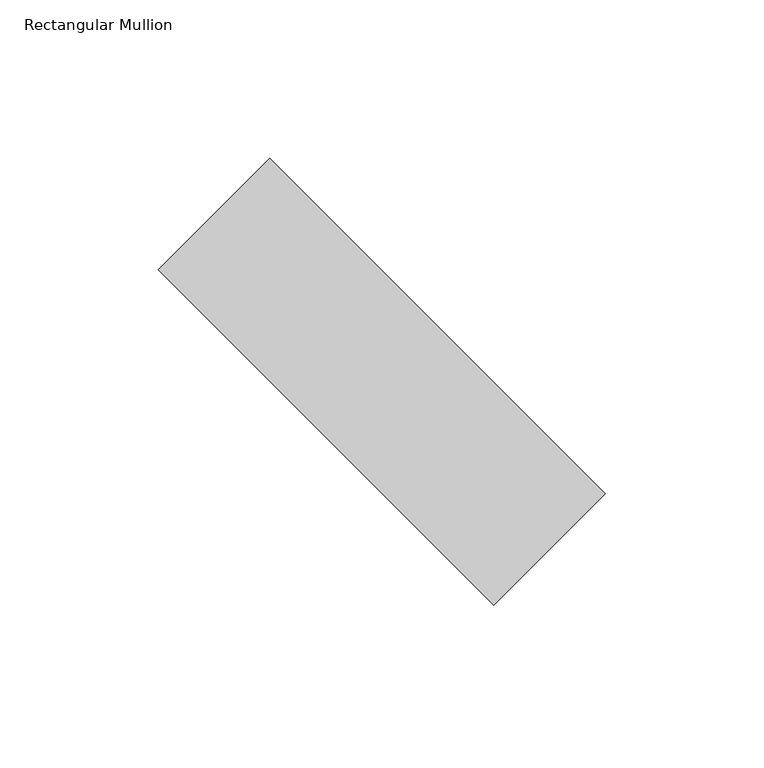
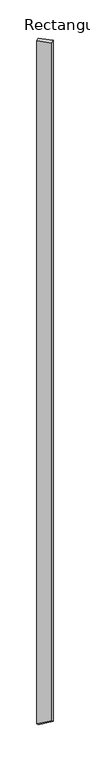
"""IFC4 building model written with IfcOpenShell, lengths in millimetres: member geometry, Rectangular Mullion : tilted mullions."""

from ifc_helpers import new_model, si_unit, origin, place, context, project, spatial, faceted_brep, source, transform, mapped, element, save


def rectangular_mullion_71da9a33(model_context):
    return source(origin(), model_context, "Body", "Brep", [
        faceted_brep([(-35.3553391, 70.7106781, 0.0), (-70.7106781, 35.3553391, 0.0), (35.3553391, -70.7106781, 0.0), (70.7106781, -35.3553391, 0.0), (-35.3553391, 70.7106781, -8054.4890214), (-70.7106781, 35.3553391, -8009.469781), (35.3553391, -70.7106781, -7944.2056108), (70.7106781, -35.3553391, -7989.2248513)], [[[0, 1, 2, 3]], [[1, 0, 4, 5]], [[2, 1, 5, 6]], [[3, 2, 6, 7]], [[0, 3, 7, 4]], [[4, 7, 6, 5]]]),
    ])


if __name__ == "__main__":
    model = new_model("IFC4")
    model_context = context("Model", 3, world=origin())
    ifc_project = project(units=[si_unit("LENGTHUNIT", "METRE", prefix="MILLI")], contexts=[model_context])
    site = spatial("IfcSite", under=ifc_project)
    building = spatial("IfcBuilding", under=site)
    placement = place(None, origin())
    rectangular_mullion_shape = rectangular_mullion_71da9a33(model_context)
    element("IfcMember", 1, ObjectType="Rectangular Mullion : tilted mullions", at=placement, inside=building, context=model_context, shape_type="MappedRepresentation", body=[
        mapped(rectangular_mullion_shape, transform((0.0, 0.0, 0.0), x_axis=(1.0, 0.0, 0.0), y_axis=(0.0, 1.0, 0.0), z_axis=(0.0, 0.0, 1.0))),
    ])
    save(model, "model.ifc")

# Revit data of these elements
# Type "Rectangular Mullion : tilted mullions"
#   built-in parameter 1007304 = 0.492126 (stored number, unit not read)
#   built-in parameter 1007301 = 0.082021 (stored number, unit not read)
#   built-in parameter 1007300 = 0.082021 (stored number, unit not read)
# Element 1 (IfcMember, "Rectangular Mullion : tilted mullions")
#   Materials on its faces: "Aluminum"
# Materials
#   "Aluminum": class "Metal", colour RGB 244 244 244, transparency 0, Description = "Aluminum 6061", Cost = 0
